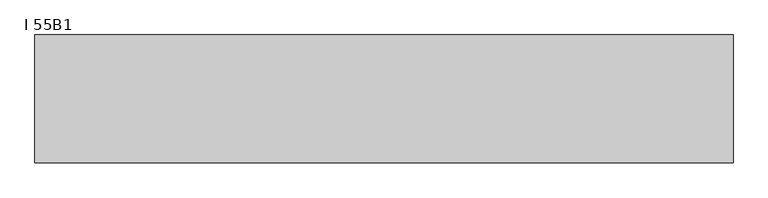
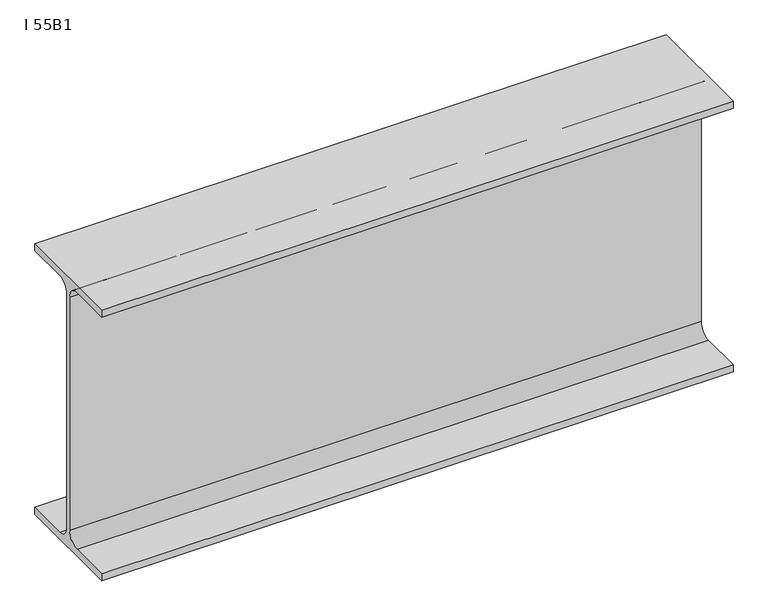
"""IFC4 building model written with IfcOpenShell, lengths in millimetres: beam geometry, Типовая двутавровая балка (АСТО 20-93) Балки : I 55B1."""

from ifc_helpers import new_model, si_unit, point, frame, frame_2d, origin, place, context, project, spatial, polyline, circle_curve, trimmed, segment, composite_curve, outline, extrude, source, transform, mapped, element, save


def i_55b1_a9d75235(model_context):
    return source(origin(), model_context, "Body", "SweptSolid", [
        extrude(outline(composite_curve([segment(polyline([(110.0, -258.0), (110.0, -271.5), (-110.0, -271.5), (-110.0, -258.0), (-28.75, -258.0)]), True, "CONTINUOUS"), segment(trimmed(circle_curve(frame_2d((-28.75, -234.0)), 24.0), [point((-28.75, -258.0))], [point((-4.75, -234.0))], True, "CARTESIAN"), True, "CONTINUOUS"), segment(polyline([(-4.75, -234.0), (-4.75, 234.0)]), True, "CONTINUOUS"), segment(trimmed(circle_curve(frame_2d((-28.75, 234.0)), 24.0), [point((-4.75, 234.0))], [point((-28.75, 258.0))], True, "CARTESIAN"), True, "CONTINUOUS"), segment(polyline([(-28.75, 258.0), (-110.0, 258.0), (-110.0, 271.5), (110.0, 271.5), (110.0, 258.0), (28.75, 258.0)]), True, "CONTINUOUS"), segment(trimmed(circle_curve(frame_2d((28.75, 234.0)), 24.0), [point((28.75, 258.0))], [point((4.75, 234.0))], True, "CARTESIAN"), True, "CONTINUOUS"), segment(polyline([(4.75, 234.0), (4.75, -234.0)]), True, "CONTINUOUS"), segment(trimmed(circle_curve(frame_2d((28.75, -234.0)), 24.0), [point((4.75, -234.0))], [point((28.75, -258.0))], True, "CARTESIAN"), True, "CONTINUOUS"), segment(polyline([(28.75, -258.0), (110.0, -258.0)]), True, "CONTINUOUS")], self_intersect=False)), frame((-600.0, 0.0, 0.0), z_axis=(1.0, 0.0, 0.0), x_axis=(0.0, 1.0, 0.0)), (0.0, 0.0, 1.0), 1200.0),
    ])


if __name__ == "__main__":
    model = new_model("IFC4")
    model_context = context("Model", 3, world=origin())
    ifc_project = project(units=[si_unit("LENGTHUNIT", "METRE", prefix="MILLI")], contexts=[model_context])
    site = spatial("IfcSite", under=ifc_project)
    building = spatial("IfcBuilding", under=site)
    placement = place(None, origin())
    i_55b1_shape = i_55b1_a9d75235(model_context)
    element("IfcBeam", 1, ObjectType="Типовая двутавровая балка (АСТО 20-93) Балки : I 55B1", at=placement, inside=building, context=model_context, shape_type="MappedRepresentation", body=[
        mapped(i_55b1_shape, transform((0.0, 0.0, 0.0), x_axis=(1.0, 0.0, 0.0), y_axis=(0.0, 1.0, 0.0), z_axis=(0.0, 0.0, 1.0))),
    ])
    save(model, "model.ifc")

# Revit data of these elements
# Type "Типовая двутавровая балка (АСТО 20-93) Балки : I 55B1"
#   ra = 24 mm
#   W = 0.872792
#   Vz = 271.5 mm
#   Vy = 110 mm
#   Vpz = 271.5 mm
#   Vpy = 110 mm
#   Length [instance default] = 1500 mm
#   bf = 220 mm
#   d = 543 mm
#   tf = 13.5 mm
#   tw = 9.5 mm
#   A = 0.011336 m²
#   Structural Material [instance default] = Металл - Сталь - 345 МПa
#   Assembly Code = ""
# Element 1 (IfcBeam, "Типовая двутавровая балка (АСТО 20-93) Балки : I 55B1")
#   Structural Material = C235
#   Materials on its faces: "C235"
# Materials
#   "Металл - Сталь - 345 МПa": class "Металл", colour RGB 247 247 247, transparency 0
#   "C235": class "Не назначено", colour RGB 0 0 0, transparency 0
